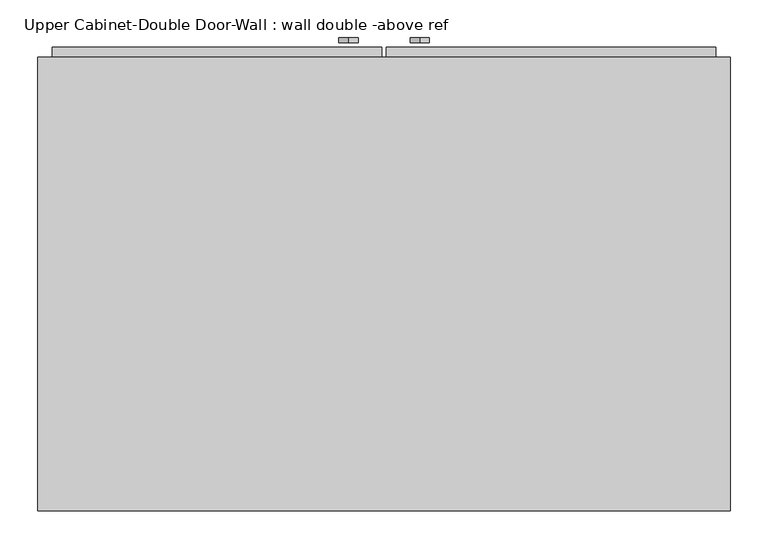
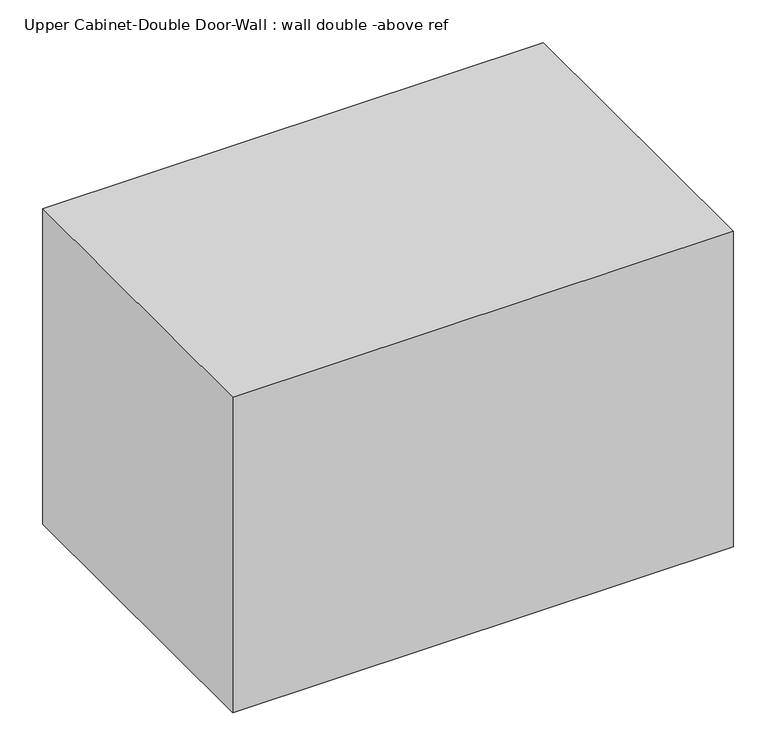
"""IFC4 building model written with IfcOpenShell, lengths in millimetres: furniture geometry, Upper Cabinet-Double Door-Wall : wall double -above ref."""

import ifcopenshell
import ifcopenshell.guid

model = None  # the IFC model being written
_history = None  # IfcOwnerHistory: only IFC2X3 demands one
_inside = {}  # id of a spatial element -> (the spatial element, [elements in it])
_under = {}  # id of a project, library or spatial element -> (it, [spatial elements below it])
_declared = {}  # id of a project -> (the project, [libraries it declares])
_typed = {}  # id of a type object -> (the type object, [elements of that type])
_made_of = {}  # id of a material, layer set ... -> (it, [elements and type objects made of it])


def new_model(schema):
    """Start an empty IFC model of exactly this schema.

    Asked for "IFC4X3", IfcOpenShell would pick the latest addendum, in which some entities
    have other attributes; the version numbers below select the first issue.
    IFC2X3 requires an IfcOwnerHistory on every rooted entity: one is made here for all.
    """
    global model, _history
    if schema == "IFC4X3":
        model = ifcopenshell.file(schema_version=(4, 3, 0, 0))
    else:
        model = ifcopenshell.file(schema=schema)
    _inside.clear()
    _under.clear()
    _declared.clear()
    _typed.clear()
    _made_of.clear()
    _history = None
    if model.schema == "IFC2X3":
        org = make("IfcOrganization", Name="unknown")
        user = make(
            "IfcPersonAndOrganization",
            ThePerson=make("IfcPerson", FamilyName="unknown"),
            TheOrganization=org,
        )
        app = make(
            "IfcApplication",
            ApplicationDeveloper=org,
            Version="unknown",
            ApplicationFullName="unknown",
            ApplicationIdentifier="unknown",
        )
        _history = make(
            "IfcOwnerHistory",
            OwningUser=user,
            OwningApplication=app,
            ChangeAction="ADDED",
            CreationDate=0,
        )
    return model


def make(cls, **values):
    """One entity of the class cls with the attributes given. An attribute that is None is left unset."""
    return model.create_entity(
        cls, **{name: value for name, value in values.items() if value is not None}
    )


def rooted(cls, **values):
    """An entity with a GlobalId (a new one), such as an element, a storey or a relation."""
    return make(cls, GlobalId=ifcopenshell.guid.new(), OwnerHistory=_history, **values)


def si_unit(unit_type, name, prefix=None):
    """IfcSIUnit, for example si_unit("LENGTHUNIT", "METRE", prefix="MILLI")."""
    return make("IfcSIUnit", UnitType=unit_type, Prefix=prefix, Name=name)


def assignment(units):
    """IfcUnitAssignment: the units of a project."""
    return None if units is None else make("IfcUnitAssignment", Units=units)


def point(xyz):
    """IfcCartesianPoint."""
    return None if xyz is None else make("IfcCartesianPoint", Coordinates=xyz)


def direction(xyz):
    """IfcDirection."""
    return None if xyz is None else make("IfcDirection", DirectionRatios=xyz)


def frame(location, z_axis=None, x_axis=None):
    """IfcAxis2Placement3D, a coordinate frame: its origin and axes. An axis left out is left unset."""
    return make(
        "IfcAxis2Placement3D",
        Location=point(location),
        Axis=direction(z_axis),
        RefDirection=direction(x_axis),
    )


def frame_2d(location, x_axis=None):
    """IfcAxis2Placement2D, a coordinate frame in the plane: its origin and x axis."""
    return make(
        "IfcAxis2Placement2D", Location=point(location), RefDirection=direction(x_axis)
    )


def origin():
    """The frame at (0, 0, 0) with its axes left unset."""
    return frame((0.0, 0.0, 0.0))


def place(relative_to, where):
    """IfcLocalPlacement: puts the frame where relative to a parent placement (None: the world)."""
    return make(
        "IfcLocalPlacement", PlacementRelTo=relative_to, RelativePlacement=where
    )


def context(
    kind, dimensions, precision=None, world=None, true_north=None, identifier=None
):
    """IfcGeometricRepresentationContext, for example the 3D "Model" context."""
    return make(
        "IfcGeometricRepresentationContext",
        ContextIdentifier=identifier,
        ContextType=kind,
        CoordinateSpaceDimension=dimensions,
        Precision=precision,
        WorldCoordinateSystem=world,
        TrueNorth=true_north,
    )


def project(units=None, contexts=None):
    """IfcProject with its units and contexts."""
    return rooted(
        "IfcProject",
        Name="project",
        RepresentationContexts=contexts,
        UnitsInContext=assignment(units),
    )


def spatial(cls, under=None, at=None, **own):
    """A site, building, storey or space (cls), placed at a placement, below another one or the project."""
    s = rooted(cls, ObjectPlacement=at, **own)
    if under is not None:
        _under.setdefault(under.id(), (under, []))[1].append(s)
    return s


def polyline(points):
    """IfcPolyline through the points."""
    return make("IfcPolyline", Points=[point(p) for p in points])


def circle_curve(where, radius):
    """IfcCircle in the frame where."""
    return make("IfcCircle", Position=where, Radius=radius)


def trimmed(basis, trim1, trim2, sense, master):
    """IfcTrimmedCurve: the piece of a basis curve between two trims."""
    return make(
        "IfcTrimmedCurve",
        BasisCurve=basis,
        Trim1=trim1,
        Trim2=trim2,
        SenseAgreement=sense,
        MasterRepresentation=master,
    )


def segment(curve, same_sense, transition):
    """IfcCompositeCurveSegment."""
    return make(
        "IfcCompositeCurveSegment",
        Transition=transition,
        SameSense=same_sense,
        ParentCurve=curve,
    )


def composite_curve(segments, self_intersect=None):
    """IfcCompositeCurve: segments joined end to end."""
    return make("IfcCompositeCurve", Segments=segments, SelfIntersect=self_intersect)


def outline(outer, holes=None, kind="AREA"):
    """IfcArbitraryClosedProfileDef: a profile drawn as a closed curve; with holes, ...WithVoids."""
    if holes is None:
        return make("IfcArbitraryClosedProfileDef", ProfileType=kind, OuterCurve=outer)
    return make(
        "IfcArbitraryProfileDefWithVoids",
        ProfileType=kind,
        OuterCurve=outer,
        InnerCurves=holes,
    )


def extrude(swept, where, along, depth):
    """IfcExtrudedAreaSolid: the profile swept, set in the frame where, extruded along a direction by depth."""
    return make(
        "IfcExtrudedAreaSolid",
        SweptArea=swept,
        Position=where,
        ExtrudedDirection=direction(along),
        Depth=depth,
    )


def faces_of(points, faces, orient=None, outer=None):
    """IfcFace entities. A face is a list of loops; a loop is a list of indices into points, from 0.

    orient and outer hold one flag for each loop. By default every Orientation is true, the
    first loop of a face is its IfcFaceOuterBound and the others are IfcFaceBound.
    """
    made = []
    for i, loops in enumerate(faces):
        bounds = []
        for j, loop in enumerate(loops):
            is_outer = j == 0 if outer is None else outer[i][j]
            bounds.append(
                make(
                    "IfcFaceOuterBound" if is_outer else "IfcFaceBound",
                    Bound=make("IfcPolyLoop", Polygon=[points[k] for k in loop]),
                    Orientation=True if orient is None else orient[i][j],
                )
            )
        made.append(make("IfcFace", Bounds=bounds))
    return made


def faceted_brep(points, faces, orient=None, outer=None, voids=None):
    """IfcFacetedBrep: a solid bounded by flat faces; with voids (closed shells), ...WithVoids."""
    shared = [point(p) for p in points]
    hull = make("IfcClosedShell", CfsFaces=faces_of(shared, faces, orient, outer))
    if voids is None:
        return make("IfcFacetedBrep", Outer=hull)
    return make(
        "IfcFacetedBrepWithVoids",
        Outer=hull,
        Voids=[
            make(cls, CfsFaces=faces_of(shared, fs, o, b)) for cls, fs, o, b in voids
        ],
    )


def shape(context_of_items, identifier, shape_type, items):
    """IfcShapeRepresentation: the items that make up one representation, for example the "Body"."""
    return make(
        "IfcShapeRepresentation",
        ContextOfItems=context_of_items,
        RepresentationIdentifier=identifier,
        RepresentationType=shape_type,
        Items=items,
    )


def source(mapping_origin, context_of_items, identifier, shape_type, items):
    """IfcRepresentationMap: a shape defined once, which mapped items show again and again."""
    return make(
        "IfcRepresentationMap",
        MappingOrigin=mapping_origin,
        MappedRepresentation=shape(context_of_items, identifier, shape_type, items),
    )


def transform(
    local_origin,
    x_axis=None,
    y_axis=None,
    z_axis=None,
    scale=None,
    scale2=None,
    scale3=None,
    uniform=True,
):
    """IfcCartesianTransformationOperator3D, or its non-uniform kind. x_axis, y_axis, z_axis: its Axis1, 2, 3."""
    if uniform:
        return make(
            "IfcCartesianTransformationOperator3D",
            Axis1=direction(x_axis),
            Axis2=direction(y_axis),
            LocalOrigin=point(local_origin),
            Scale=scale,
            Axis3=direction(z_axis),
        )
    return make(
        "IfcCartesianTransformationOperator3DnonUniform",
        Axis1=direction(x_axis),
        Axis2=direction(y_axis),
        LocalOrigin=point(local_origin),
        Scale=scale,
        Axis3=direction(z_axis),
        Scale2=scale2,
        Scale3=scale3,
    )


def mapped(mapping_source, mapping_target):
    """IfcMappedItem: shows the shape of a source again, moved by a transform."""
    return make(
        "IfcMappedItem", MappingSource=mapping_source, MappingTarget=mapping_target
    )


def made_of(thing, what):
    """Note that an element or type object is made of a material, layer set ...; save() writes the relation."""
    if what is not None:
        _made_of.setdefault(what.id(), (what, []))[1].append(thing)
    return thing


def element(
    cls,
    number,
    at=None,
    inside=None,
    cuts=None,
    type_object=None,
    material=None,
    context=None,
    identifier="Body",
    shape_type=None,
    held_by="IfcProductDefinitionShape",
    body=None,
    shapes=None,
    **own,
):
    """One element of the class cls, such as IfcWall. Its Tag is "e" and its number.

    at: its placement. inside: the storey or other place that contains it. cuts: it is an
    opening in that element (IfcRelVoidsElement). A single representation is given by context,
    identifier, shape_type and body (its items); several are given by shapes. held_by: the class
    of the entity that holds the representations. save() writes the other relations.
    """
    e = rooted(cls, Tag="e%d" % number, ObjectPlacement=at, **own)
    if body is not None:
        shapes = [shape(context, identifier, shape_type, body)]
    if shapes is not None:
        e.Representation = make(held_by, Representations=shapes)
    if inside is not None:
        _inside.setdefault(inside.id(), (inside, []))[1].append(e)
    if cuts is not None:
        rooted(
            "IfcRelVoidsElement", RelatingBuildingElement=cuts, RelatedOpeningElement=e
        )
    if type_object is not None:
        _typed.setdefault(type_object.id(), (type_object, []))[1].append(e)
    return made_of(e, material)


def aggregate(whole, parts):
    """IfcRelAggregates: a whole, such as a stair, and the parts it consists of."""
    return rooted("IfcRelAggregates", RelatingObject=whole, RelatedObjects=parts)


def save(model, path):
    """Write the relations noted so far, then the file.

    IfcRelAggregates (storeys below a building ...), IfcRelContainedInSpatialStructure (elements
    in a storey), IfcRelDefinesByType, IfcRelAssociatesMaterial and IfcRelDeclares: one each for
    every whole, place, type object, material and project.
    """
    for whole, parts in _under.values():
        aggregate(whole, parts)
    for where, things in _inside.values():
        rooted(
            "IfcRelContainedInSpatialStructure",
            RelatedElements=things,
            RelatingStructure=where,
        )
    for kind, things in _typed.values():
        rooted("IfcRelDefinesByType", RelatedObjects=things, RelatingType=kind)
    for what, things in _made_of.values():
        rooted("IfcRelAssociatesMaterial", RelatedObjects=things, RelatingMaterial=what)
    for by, libraries in _declared.values():
        rooted("IfcRelDeclares", RelatingContext=by, RelatedDefinitions=libraries)
    model.write(path)


def upper_cabinet_double_door_wall_wall_double_above_ref_e0faee37(model_context):
    return source(origin(), model_context, "Body", "SolidModel", [
        faceted_brep([(-427.4288372, 57.15, 2133.6), (-427.4288372, 57.15, 1524.0), (486.9711628, 57.15, 1524.0), (486.9711628, 57.15, 2133.6), (-427.4288372, 657.1257812, 2133.6), (486.9711628, 657.1257812, 2133.6), (486.9711628, 657.1257812, 1524.0), (-427.4288372, 657.1257812, 1524.0), (-408.3788372, 657.1257812, 2114.55), (-408.3788372, 657.1257812, 1543.05), (467.9211628, 657.1257812, 1543.05), (467.9211628, 657.1257812, 2114.55), (467.9211628, 76.2, 2114.55), (-408.3788372, 76.2, 2114.55), (467.9211628, 76.2, 1543.05), (-408.3788372, 76.2, 1543.05)], [[[0, 1, 2, 3]], [[4, 5, 6, 7], [8, 9, 10, 11]], [[1, 0, 4, 7]], [[2, 1, 7, 6]], [[3, 2, 6, 5]], [[0, 3, 5, 4]], [[8, 11, 12, 13]], [[11, 10, 14, 12]], [[10, 9, 15, 14]], [[9, 8, 13, 15]], [[13, 12, 14, 15]]]),
        extrude(outline(polyline([(32.9461628, 669.8257813), (467.9211628, 669.8257813), (467.9211628, 638.0757813), (32.9461628, 638.0757813), (32.9461628, 669.8257813)])), frame((0.0, 0.0, 1543.05), z_axis=(0.0, 0.0, 1.0), x_axis=(1.0, 0.0, 0.0)), (0.0, 0.0, 1.0), 571.5),
        extrude(outline(polyline([(-408.3788372, 669.8257813), (26.5961628, 669.8257813), (26.5961628, 638.0757813), (-408.3788372, 638.0757813), (-408.3788372, 669.8257813)])), frame((0.0, 0.0, 1543.05), z_axis=(0.0, 0.0, 1.0), x_axis=(1.0, 0.0, 0.0)), (0.0, 0.0, 1.0), 571.5),
        extrude(outline(composite_curve([segment(trimmed(circle_curve(frame_2d((1686.2214732, 76.8007051)), 12.7), [point((1673.5214732, 76.8007051))], [point((1698.9214732, 76.8007051))], False, "CARTESIAN"), True, "CONTINUOUS"), segment(trimmed(circle_curve(frame_2d((1686.2214732, 76.8007051)), 12.7), [point((1698.9214732, 76.8007051))], [point((1673.5214732, 76.8007051))], False, "CARTESIAN"), True, "CONTINUOUS")], self_intersect=False)), frame((0.0, 676.1757813, 0.0), z_axis=(0.0, 1.0, 0.0), x_axis=(0.0, 0.0, 1.0)), (0.0, 0.0, 1.0), 6.35),
        extrude(outline(composite_curve([segment(trimmed(circle_curve(frame_2d((1686.2214732, -17.2583796)), 12.7), [point((1673.5214732, -17.2583796))], [point((1698.9214732, -17.2583796))], False, "CARTESIAN"), True, "CONTINUOUS"), segment(trimmed(circle_curve(frame_2d((1686.2214732, -17.2583796)), 12.7), [point((1698.9214732, -17.2583796))], [point((1673.5214732, -17.2583796))], False, "CARTESIAN"), True, "CONTINUOUS")], self_intersect=False)), frame((0.0, 676.1757813, 0.0), z_axis=(0.0, 1.0, 0.0), x_axis=(0.0, 0.0, 1.0)), (0.0, 0.0, 1.0), 6.35),
    ])


if __name__ == "__main__":
    model = new_model("IFC4")
    model_context = context("Model", 3, world=origin())
    ifc_project = project(units=[si_unit("LENGTHUNIT", "METRE", prefix="MILLI")], contexts=[model_context])
    site = spatial("IfcSite", under=ifc_project)
    building = spatial("IfcBuilding", under=site)
    placement = place(None, origin())
    upper_cabinet_double_door_wall_wall_double_above_ref_shape = upper_cabinet_double_door_wall_wall_double_above_ref_e0faee37(model_context)
    element("IfcFurniture", 1, ObjectType="Upper Cabinet-Double Door-Wall : wall double -above ref", at=placement, inside=building, context=model_context, shape_type="MappedRepresentation", body=[
        mapped(upper_cabinet_double_door_wall_wall_double_above_ref_shape, transform((0.0, 0.0, 0.0), x_axis=(1.0, 0.0, 0.0), y_axis=(0.0, 1.0, 0.0), z_axis=(0.0, 0.0, 1.0))),
    ])
    save(model, "model.ifc")

# Revit data of these elements
# Type "Upper Cabinet-Double Door-Wall : wall double -above ref"
#   Assembly Code = "C1030410"
#   Depth = 1' - 11 159/256"
#   Height = 2' - 0"
#   Top Of Cabinet = 7' - 0"
#   Width = 3' - 0"
#   Cabinet Material = Base cabinet 2120100 Aspekt - 83012120100 - White
#   Door/Drawer Material = Base cabinet 2120100 Aspekt - 83012120100 - White
#   Handle Material = Cabinets - Handles
#   Default Elevation = 0
# Element 1 (IfcFurniture, "Upper Cabinet-Double Door-Wall : wall double -above ref")
#   Materials on its faces: "Base cabinet 2120100 Aspekt - 83012120100 - White"
# Materials
#   "Base cabinet 2120100 Aspekt - 83012120100 - White": class "Miscellaneous", colour RGB 255 255 255, transparency 0, Manufacturer = "Marbodal", URL = "http://www.marbodal.se", Cost = 0
#   "Cabinets - Handles": class "Metal", colour RGB 57 57 57, transparency 0
